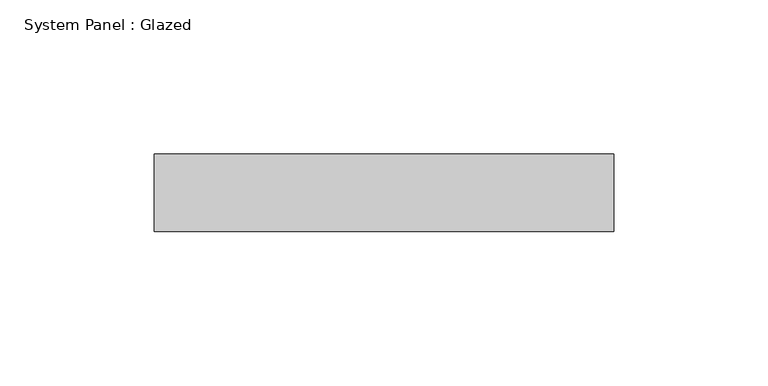
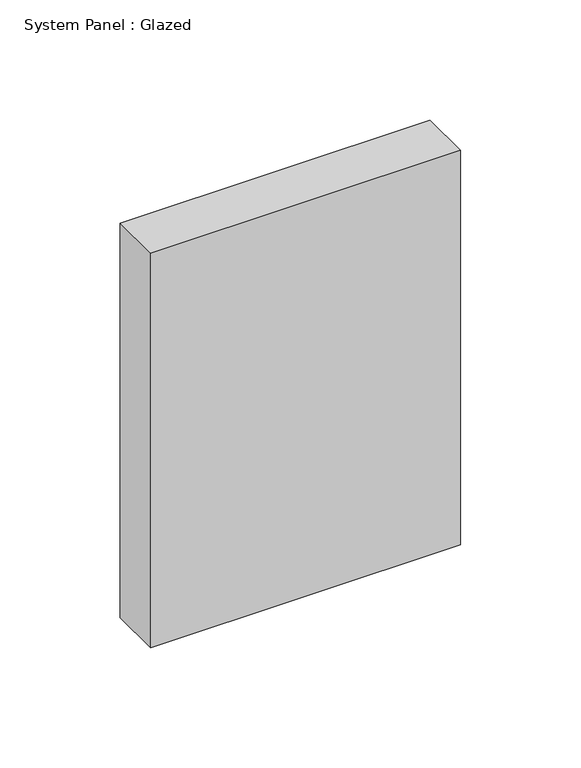
"""IFC4 building model written with IfcOpenShell, lengths in millimetres: plate geometry, System Panel : Glazed."""

from ifc_helpers import new_model, si_unit, origin, origin_with_axes, place, context, project, spatial, polyline, outline, extrude, source, transform, mapped, element, save


def system_panel_glazed_937a8ef3(model_context):
    return source(origin(), model_context, "Body", "SweptSolid", [
        extrude(outline(polyline([(74.3295665, 24.5), (-74.3295665, 24.5), (-74.3295665, 49.5), (74.3295665, 49.5), (74.3295665, 24.5)])), origin_with_axes(), (0.0, 0.0, 1.0), 200.0),
    ])


if __name__ == "__main__":
    model = new_model("IFC4")
    model_context = context("Model", 3, world=origin())
    ifc_project = project(units=[si_unit("LENGTHUNIT", "METRE", prefix="MILLI")], contexts=[model_context])
    site = spatial("IfcSite", under=ifc_project)
    building = spatial("IfcBuilding", under=site)
    placement = place(None, origin())
    system_panel_glazed_shape = system_panel_glazed_937a8ef3(model_context)
    element("IfcPlate", 1, ObjectType="System Panel : Glazed", at=placement, inside=building, context=model_context, shape_type="MappedRepresentation", body=[
        mapped(system_panel_glazed_shape, transform((0.0, 0.0, 0.0), x_axis=(1.0, 0.0, 0.0), y_axis=(0.0, 1.0, 0.0), z_axis=(0.0, 0.0, 1.0))),
    ])
    save(model, "model.ifc")

# Revit data of these elements
# Element 1 (IfcPlate, "System Panel : Glazed")
#   Materials on its faces: "Glass"
# Materials
#   "Glass": class "Glass", colour RGB 218 227 224, transparency 0.85, Description = "Soda Lime Glass", Cost = 0
